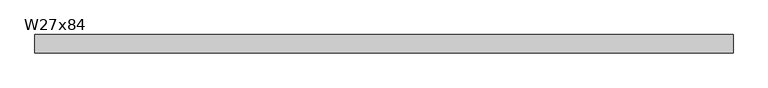
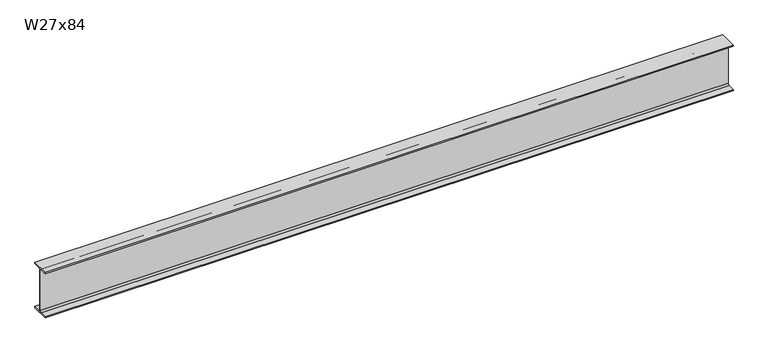
"""IFC4 building model written with IfcOpenShell, lengths in millimetres: beam geometry, RME W-Wide Flange : W27x84."""

from ifc_helpers import new_model, si_unit, point, frame, frame_2d, origin, place, context, project, spatial, polyline, circle_curve, trimmed, segment, composite_curve, outline, extrude, source, transform, mapped, element, save


def w27x84_956fdd2e(model_context):
    return source(origin(), model_context, "Body", "SweptSolid", [
        extrude(outline(composite_curve([segment(polyline([(127.0, -322.834), (127.0, -339.09), (-127.0, -339.09), (-127.0, -322.834), (-29.2735, -322.834)]), True, "CONTINUOUS"), segment(trimmed(circle_curve(frame_2d((-29.2735, -299.4025)), 23.4315), [point((-29.2735, -322.834))], [point((-5.842, -299.4025))], True, "CARTESIAN"), True, "CONTINUOUS"), segment(polyline([(-5.842, -299.4025), (-5.842, 299.4025)]), True, "CONTINUOUS"), segment(trimmed(circle_curve(frame_2d((-29.2735, 299.4025)), 23.4315), [point((-5.842, 299.4025))], [point((-29.2735, 322.834))], True, "CARTESIAN"), True, "CONTINUOUS"), segment(polyline([(-29.2735, 322.834), (-127.0, 322.834), (-127.0, 339.09), (127.0, 339.09), (127.0, 322.834), (29.2735, 322.834)]), True, "CONTINUOUS"), segment(trimmed(circle_curve(frame_2d((29.2735, 299.4025)), 23.4315), [point((29.2735, 322.834))], [point((5.842, 299.4025))], True, "CARTESIAN"), True, "CONTINUOUS"), segment(polyline([(5.842, 299.4025), (5.842, -299.4025)]), True, "CONTINUOUS"), segment(trimmed(circle_curve(frame_2d((29.2735, -299.4025)), 23.4315), [point((5.842, -299.4025))], [point((29.2735, -322.834))], True, "CARTESIAN"), True, "CONTINUOUS"), segment(polyline([(29.2735, -322.834), (127.0, -322.834)]), True, "CONTINUOUS")], self_intersect=False)), frame((-4858.541454, 0.0, 0.0), z_axis=(1.0, 0.0, 0.0), x_axis=(0.0, 1.0, 0.0)), (0.0, 0.0, 1.0), 9717.0829081),
    ])


if __name__ == "__main__":
    model = new_model("IFC4")
    model_context = context("Model", 3, world=origin())
    ifc_project = project(units=[si_unit("LENGTHUNIT", "METRE", prefix="MILLI")], contexts=[model_context])
    site = spatial("IfcSite", under=ifc_project)
    building = spatial("IfcBuilding", under=site)
    placement = place(None, origin())
    w27x84_shape = w27x84_956fdd2e(model_context)
    element("IfcBeam", 1, ObjectType="RME W-Wide Flange : W27x84", at=placement, inside=building, context=model_context, shape_type="MappedRepresentation", body=[
        mapped(w27x84_shape, transform((0.0, 0.0, 0.0), x_axis=(1.0, 0.0, 0.0), y_axis=(0.0, 1.0, 0.0), z_axis=(0.0, 0.0, 1.0))),
    ])
    save(model, "model.ifc")

# Revit data of these elements
# Type "RME W-Wide Flange : W27x84"
#   WELD P [instance default] = ""
#   WELD LE [instance default] = ""
#   WELD D [instance default] = ""
#   TOP SECTION SIZE [instance default] = ""
#   TOP SECTION LENGTH [instance default] = ""
#   REMARKS [instance default] = ""
#   REINF TYPE [instance default] = ""
#   Nominal Size = "W24"
#   End Bearing Capacity [instance default] = ""
#   BOT SECTION SIZE [instance default] = ""
#   BOT SECTION LENGTH [instance default] = ""
#   Assembly Code = "B10"
#   W = 84
#   Start Extension Calculation [instance default] = 10' - 0"
#   Start Extension [instance default] = -0' - 0 1/2"
#   End Extension Calculation [instance default] = 10' - 0"
#   End Extension [instance default] = -0' - 0 1/2"
#   Length [instance default] = 5' - 0"
#   bf = 0' - 10"
#   d = 2' - 2.7"
#   k = 0' - 1 9/16"
#   k2 = 0' - 0.9225"
#   tf = 0' - 0.64"
#   tw = 0' - 0.46"
#   A = 0.172222 SF
#   Structural Material [instance default] = Metal - Steel - ASTM A992
# Element 1 (IfcBeam, "RME W-Wide Flange : W27x84")
#   Length = 32' - 7.49232"
#   Materials on its faces: "Metal - Steel - ASTM A992"
# Materials
#   "Metal - Steel - ASTM A992": class "Metal", colour RGB 255 128 0, transparency 0
